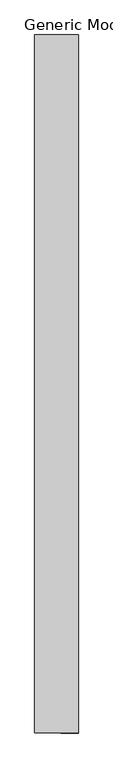
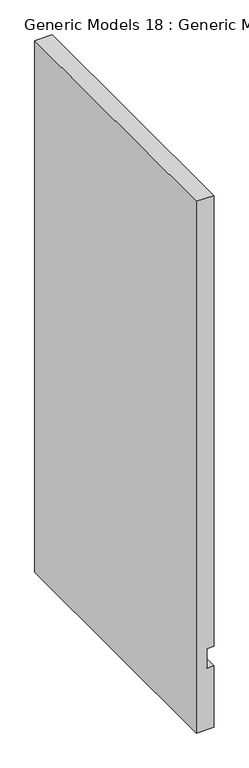
"""IFC4 building model written with IfcOpenShell, lengths in millimetres: proxy geometry, Generic Models 18 : Generic Models 1."""

import ifcopenshell
import ifcopenshell.guid

model = None  # the IFC model being written
_history = None  # IfcOwnerHistory: only IFC2X3 demands one
_inside = {}  # id of a spatial element -> (the spatial element, [elements in it])
_under = {}  # id of a project, library or spatial element -> (it, [spatial elements below it])
_declared = {}  # id of a project -> (the project, [libraries it declares])
_typed = {}  # id of a type object -> (the type object, [elements of that type])
_made_of = {}  # id of a material, layer set ... -> (it, [elements and type objects made of it])


def new_model(schema):
    """Start an empty IFC model of exactly this schema.

    Asked for "IFC4X3", IfcOpenShell would pick the latest addendum, in which some entities
    have other attributes; the version numbers below select the first issue.
    IFC2X3 requires an IfcOwnerHistory on every rooted entity: one is made here for all.
    """
    global model, _history
    if schema == "IFC4X3":
        model = ifcopenshell.file(schema_version=(4, 3, 0, 0))
    else:
        model = ifcopenshell.file(schema=schema)
    _inside.clear()
    _under.clear()
    _declared.clear()
    _typed.clear()
    _made_of.clear()
    _history = None
    if model.schema == "IFC2X3":
        org = make("IfcOrganization", Name="unknown")
        user = make(
            "IfcPersonAndOrganization",
            ThePerson=make("IfcPerson", FamilyName="unknown"),
            TheOrganization=org,
        )
        app = make(
            "IfcApplication",
            ApplicationDeveloper=org,
            Version="unknown",
            ApplicationFullName="unknown",
            ApplicationIdentifier="unknown",
        )
        _history = make(
            "IfcOwnerHistory",
            OwningUser=user,
            OwningApplication=app,
            ChangeAction="ADDED",
            CreationDate=0,
        )
    return model


def make(cls, **values):
    """One entity of the class cls with the attributes given. An attribute that is None is left unset."""
    return model.create_entity(
        cls, **{name: value for name, value in values.items() if value is not None}
    )


def rooted(cls, **values):
    """An entity with a GlobalId (a new one), such as an element, a storey or a relation."""
    return make(cls, GlobalId=ifcopenshell.guid.new(), OwnerHistory=_history, **values)


def si_unit(unit_type, name, prefix=None):
    """IfcSIUnit, for example si_unit("LENGTHUNIT", "METRE", prefix="MILLI")."""
    return make("IfcSIUnit", UnitType=unit_type, Prefix=prefix, Name=name)


def assignment(units):
    """IfcUnitAssignment: the units of a project."""
    return None if units is None else make("IfcUnitAssignment", Units=units)


def point(xyz):
    """IfcCartesianPoint."""
    return None if xyz is None else make("IfcCartesianPoint", Coordinates=xyz)


def direction(xyz):
    """IfcDirection."""
    return None if xyz is None else make("IfcDirection", DirectionRatios=xyz)


def frame(location, z_axis=None, x_axis=None):
    """IfcAxis2Placement3D, a coordinate frame: its origin and axes. An axis left out is left unset."""
    return make(
        "IfcAxis2Placement3D",
        Location=point(location),
        Axis=direction(z_axis),
        RefDirection=direction(x_axis),
    )


def origin():
    """The frame at (0, 0, 0) with its axes left unset."""
    return frame((0.0, 0.0, 0.0))


def place(relative_to, where):
    """IfcLocalPlacement: puts the frame where relative to a parent placement (None: the world)."""
    return make(
        "IfcLocalPlacement", PlacementRelTo=relative_to, RelativePlacement=where
    )


def context(
    kind, dimensions, precision=None, world=None, true_north=None, identifier=None
):
    """IfcGeometricRepresentationContext, for example the 3D "Model" context."""
    return make(
        "IfcGeometricRepresentationContext",
        ContextIdentifier=identifier,
        ContextType=kind,
        CoordinateSpaceDimension=dimensions,
        Precision=precision,
        WorldCoordinateSystem=world,
        TrueNorth=true_north,
    )


def project(units=None, contexts=None):
    """IfcProject with its units and contexts."""
    return rooted(
        "IfcProject",
        Name="project",
        RepresentationContexts=contexts,
        UnitsInContext=assignment(units),
    )


def spatial(cls, under=None, at=None, **own):
    """A site, building, storey or space (cls), placed at a placement, below another one or the project."""
    s = rooted(cls, ObjectPlacement=at, **own)
    if under is not None:
        _under.setdefault(under.id(), (under, []))[1].append(s)
    return s


def polyline(points):
    """IfcPolyline through the points."""
    return make("IfcPolyline", Points=[point(p) for p in points])


def outline(outer, holes=None, kind="AREA"):
    """IfcArbitraryClosedProfileDef: a profile drawn as a closed curve; with holes, ...WithVoids."""
    if holes is None:
        return make("IfcArbitraryClosedProfileDef", ProfileType=kind, OuterCurve=outer)
    return make(
        "IfcArbitraryProfileDefWithVoids",
        ProfileType=kind,
        OuterCurve=outer,
        InnerCurves=holes,
    )


def extrude(swept, where, along, depth):
    """IfcExtrudedAreaSolid: the profile swept, set in the frame where, extruded along a direction by depth."""
    return make(
        "IfcExtrudedAreaSolid",
        SweptArea=swept,
        Position=where,
        ExtrudedDirection=direction(along),
        Depth=depth,
    )


def shape(context_of_items, identifier, shape_type, items):
    """IfcShapeRepresentation: the items that make up one representation, for example the "Body"."""
    return make(
        "IfcShapeRepresentation",
        ContextOfItems=context_of_items,
        RepresentationIdentifier=identifier,
        RepresentationType=shape_type,
        Items=items,
    )


def source(mapping_origin, context_of_items, identifier, shape_type, items):
    """IfcRepresentationMap: a shape defined once, which mapped items show again and again."""
    return make(
        "IfcRepresentationMap",
        MappingOrigin=mapping_origin,
        MappedRepresentation=shape(context_of_items, identifier, shape_type, items),
    )


def transform(
    local_origin,
    x_axis=None,
    y_axis=None,
    z_axis=None,
    scale=None,
    scale2=None,
    scale3=None,
    uniform=True,
):
    """IfcCartesianTransformationOperator3D, or its non-uniform kind. x_axis, y_axis, z_axis: its Axis1, 2, 3."""
    if uniform:
        return make(
            "IfcCartesianTransformationOperator3D",
            Axis1=direction(x_axis),
            Axis2=direction(y_axis),
            LocalOrigin=point(local_origin),
            Scale=scale,
            Axis3=direction(z_axis),
        )
    return make(
        "IfcCartesianTransformationOperator3DnonUniform",
        Axis1=direction(x_axis),
        Axis2=direction(y_axis),
        LocalOrigin=point(local_origin),
        Scale=scale,
        Axis3=direction(z_axis),
        Scale2=scale2,
        Scale3=scale3,
    )


def mapped(mapping_source, mapping_target):
    """IfcMappedItem: shows the shape of a source again, moved by a transform."""
    return make(
        "IfcMappedItem", MappingSource=mapping_source, MappingTarget=mapping_target
    )


def made_of(thing, what):
    """Note that an element or type object is made of a material, layer set ...; save() writes the relation."""
    if what is not None:
        _made_of.setdefault(what.id(), (what, []))[1].append(thing)
    return thing


def element(
    cls,
    number,
    at=None,
    inside=None,
    cuts=None,
    type_object=None,
    material=None,
    context=None,
    identifier="Body",
    shape_type=None,
    held_by="IfcProductDefinitionShape",
    body=None,
    shapes=None,
    **own,
):
    """One element of the class cls, such as IfcWall. Its Tag is "e" and its number.

    at: its placement. inside: the storey or other place that contains it. cuts: it is an
    opening in that element (IfcRelVoidsElement). A single representation is given by context,
    identifier, shape_type and body (its items); several are given by shapes. held_by: the class
    of the entity that holds the representations. save() writes the other relations.
    """
    e = rooted(cls, Tag="e%d" % number, ObjectPlacement=at, **own)
    if body is not None:
        shapes = [shape(context, identifier, shape_type, body)]
    if shapes is not None:
        e.Representation = make(held_by, Representations=shapes)
    if inside is not None:
        _inside.setdefault(inside.id(), (inside, []))[1].append(e)
    if cuts is not None:
        rooted(
            "IfcRelVoidsElement", RelatingBuildingElement=cuts, RelatedOpeningElement=e
        )
    if type_object is not None:
        _typed.setdefault(type_object.id(), (type_object, []))[1].append(e)
    return made_of(e, material)


def aggregate(whole, parts):
    """IfcRelAggregates: a whole, such as a stair, and the parts it consists of."""
    return rooted("IfcRelAggregates", RelatingObject=whole, RelatedObjects=parts)


def save(model, path):
    """Write the relations noted so far, then the file.

    IfcRelAggregates (storeys below a building ...), IfcRelContainedInSpatialStructure (elements
    in a storey), IfcRelDefinesByType, IfcRelAssociatesMaterial and IfcRelDeclares: one each for
    every whole, place, type object, material and project.
    """
    for whole, parts in _under.values():
        aggregate(whole, parts)
    for where, things in _inside.values():
        rooted(
            "IfcRelContainedInSpatialStructure",
            RelatedElements=things,
            RelatingStructure=where,
        )
    for kind, things in _typed.values():
        rooted("IfcRelDefinesByType", RelatedObjects=things, RelatingType=kind)
    for what, things in _made_of.values():
        rooted("IfcRelAssociatesMaterial", RelatedObjects=things, RelatingMaterial=what)
    for by, libraries in _declared.values():
        rooted("IfcRelDeclares", RelatingContext=by, RelatedDefinitions=libraries)
    model.write(path)


def generic_models_18_generic_models_1_971eb1a3(model_context):
    return source(origin(), model_context, "Body", "SweptSolid", [
        extrude(outline(polyline([(7.9375, 49699.8625), (7.9375, 49776.0625), (291.1195631, 49776.0625), (291.1195631, 49745.9), (380.0195631, 49745.9), (380.0195631, 49776.0625), (2452.6875, 49776.0625), (2452.6875, 49699.8625), (7.9375, 49699.8625)])), frame((0.0, 0.0, 0.0), z_axis=(0.0, 1.0, 0.0), x_axis=(0.0, 0.0, 1.0)), (0.0, 0.0, 1.0), 1219.2),
    ])


if __name__ == "__main__":
    model = new_model("IFC4")
    model_context = context("Model", 3, world=origin())
    ifc_project = project(units=[si_unit("LENGTHUNIT", "METRE", prefix="MILLI")], contexts=[model_context])
    site = spatial("IfcSite", under=ifc_project)
    building = spatial("IfcBuilding", under=site)
    placement = place(None, origin())
    generic_models_18_generic_models_1_shape = generic_models_18_generic_models_1_971eb1a3(model_context)
    element("IfcBuildingElementProxy", 1, Name="Generic Models 18 : Generic Models 1", ObjectType="Generic Models 18 : Generic Models 1", at=placement, inside=building, context=model_context, shape_type="MappedRepresentation", body=[
        mapped(generic_models_18_generic_models_1_shape, transform((0.0, 0.0, 0.0), x_axis=(1.0, 0.0, 0.0), y_axis=(0.0, 1.0, 0.0), z_axis=(0.0, 0.0, 1.0))),
    ])
    save(model, "model.ifc")

# Revit data of these elements
# Element 1 (IfcBuildingElementProxy, "Generic Models 18 : Generic Models 1")
#   Materials on its faces: "(S) SOUND BATT. INSULATION (THICKNESS TO MATCH WALL DEPTH)"
# Materials
#   "(S) SOUND BATT. INSULATION (THICKNESS TO MATCH WALL DEPTH)": class "Unassigned", colour RGB 255 255 255, transparency 0, Cost = 0
